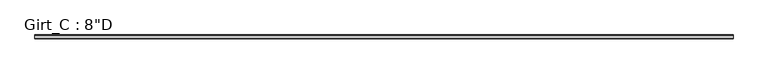
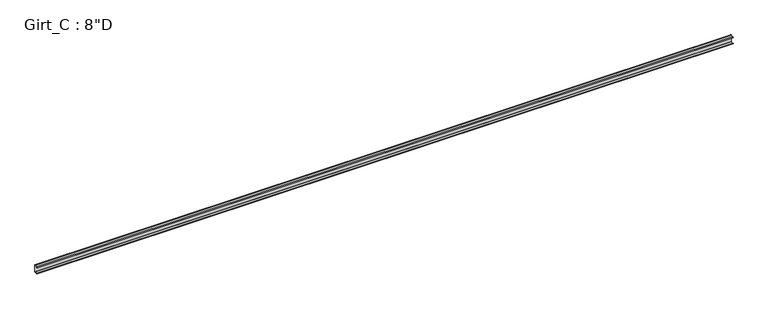
"""IFC4 building model written with IfcOpenShell, lengths in millimetres: beam geometry."""

from ifc_helpers import new_model, si_unit, point, frame, frame_2d, origin, place, context, project, spatial, polyline, circle_curve, trimmed, segment, composite_curve, outline, extrude, source, transform, mapped, element, save


def beam_9edf529d(model_context):
    return source(origin(), model_context, "Body", "SweptSolid", [
        extrude(outline(composite_curve([segment(polyline([(-87.5109375, 101.6), (-3.3734375, 101.6)]), True, "CONTINUOUS"), segment(trimmed(circle_curve(frame_2d((-3.3734375, 96.8375)), 4.7625), [point((-3.3734375, 101.6))], [point((1.3890625, 96.8375))], False, "CARTESIAN"), True, "CONTINUOUS"), segment(polyline([(1.3890625, 96.8375), (1.3890625, -96.8375)]), True, "CONTINUOUS"), segment(trimmed(circle_curve(frame_2d((-3.3734375, -96.8375)), 4.7625), [point((1.3890625, -96.8375))], [point((-3.3734375, -101.6))], False, "CARTESIAN"), True, "CONTINUOUS"), segment(polyline([(-3.3734375, -101.6), (-87.5109375, -101.6), (-99.7792647, -86.979177), (-97.6510975, -85.1934327), (-86.2154765, -98.821875), (-3.2694106, -98.821875)]), True, "CONTINUOUS"), segment(trimmed(circle_curve(frame_2d((-3.3748024, -96.8389339)), 1.9857399), [point((-3.2694106, -98.821875))], [point((-1.3890625, -96.8389339))], True, "CARTESIAN"), True, "CONTINUOUS"), segment(polyline([(-1.3890625, -96.8389339), (-1.3890625, 96.8381931)]), True, "CONTINUOUS"), segment(trimmed(circle_curve(frame_2d((-3.3741066, 96.8381931)), 1.9850441), [point((-1.3890625, 96.8381931))], [point((-3.3005807, 98.821875))], True, "CARTESIAN"), True, "CONTINUOUS"), segment(polyline([(-3.3005807, 98.821875), (-86.2154765, 98.821875), (-97.6278742, 85.221109), (-99.7560415, 87.0068534), (-87.5109375, 101.6)]), True, "CONTINUOUS")], self_intersect=False)), frame((-9256.8059343, 0.0, 0.0), z_axis=(1.0, 0.0, 0.0), x_axis=(0.0, 1.0, 0.0)), (0.0, 0.0, 1.0), 19092.545),
    ])


if __name__ == "__main__":
    model = new_model("IFC4")
    model_context = context("Model", 3, world=origin())
    ifc_project = project(units=[si_unit("LENGTHUNIT", "METRE", prefix="MILLI")], contexts=[model_context])
    site = spatial("IfcSite", under=ifc_project)
    building = spatial("IfcBuilding", under=site)
    placement = place(None, origin())
    beam_shape = beam_9edf529d(model_context)
    element("IfcBeam", 1, ObjectType="Girt_C : 8\"D", at=placement, inside=building, context=model_context, shape_type="MappedRepresentation", body=[
        mapped(beam_shape, transform((0.0, 0.0, 0.0), x_axis=(1.0, 0.0, 0.0), y_axis=(0.0, 1.0, 0.0), z_axis=(0.0, 0.0, 1.0))),
    ])
    save(model, "model.ifc")

# Revit data of these elements
# Type "Girt_C : 8\"D"
#   half leg = 0' - 1 3/4"
#   Web_Thickness = 0' - 0 7/64"
#   Length [instance default] = 10' - 0"
#   Leg_1 = 0' - 3 1/2"
#   Height = 0' - 8"
#   Structural Material [instance default] = none
# Element 1 (IfcBeam, "Girt_C : 8\"D")
#   Structural Material = CEE' SECTION (8.0x3.5C - SEE STRUCT. DWGS)
#   Materials on its faces: "CEE' SECTION (8.0x3.5C - SEE STRUCT. DWGS)"
# Materials
#   "CEE' SECTION (8.0x3.5C - SEE STRUCT. DWGS)": class "Metal", colour RGB 137 146 153, transparency 0, Description = "Steel, mill finish", Cost = 0
